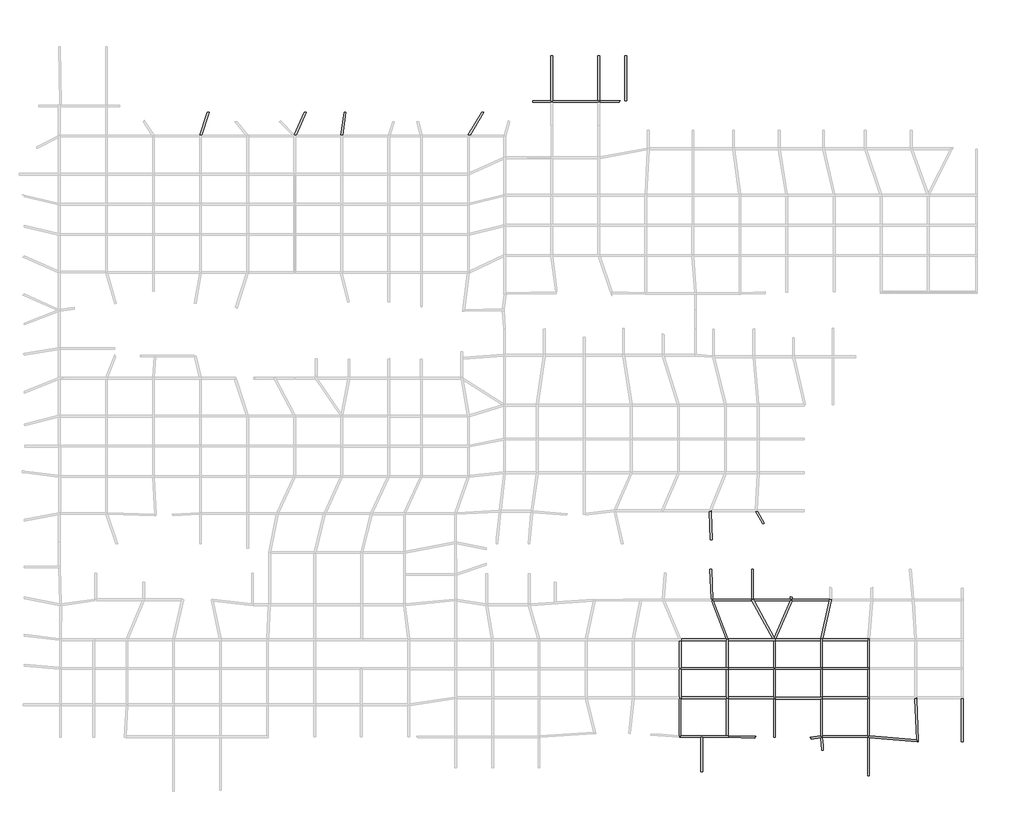
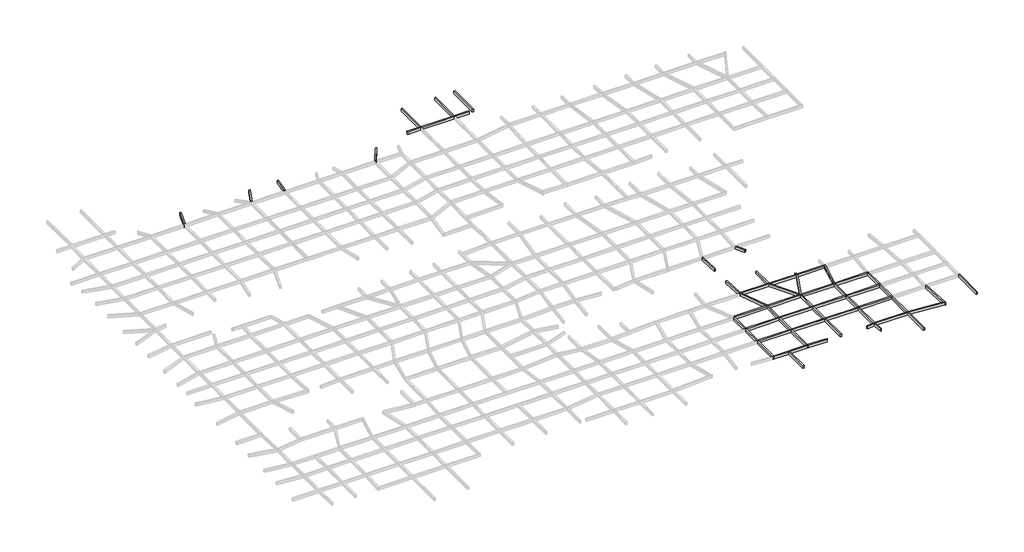
# One storey, part 13 of 15: 59 beams.
"""IFC4 building model written with IfcOpenShell, lengths in millimetres."""

import ifcopenshell
import ifcopenshell.guid

model = None  # the IFC model being written
_history = None  # IfcOwnerHistory: only IFC2X3 demands one
_inside = {}  # id of a spatial element -> (the spatial element, [elements in it])
_under = {}  # id of a project, library or spatial element -> (it, [spatial elements below it])
_declared = {}  # id of a project -> (the project, [libraries it declares])
_typed = {}  # id of a type object -> (the type object, [elements of that type])
_made_of = {}  # id of a material, layer set ... -> (it, [elements and type objects made of it])


def new_model(schema):
    """Start an empty IFC model of exactly this schema.

    Asked for "IFC4X3", IfcOpenShell would pick the latest addendum, in which some entities
    have other attributes; the version numbers below select the first issue.
    IFC2X3 requires an IfcOwnerHistory on every rooted entity: one is made here for all.
    """
    global model, _history
    if schema == "IFC4X3":
        model = ifcopenshell.file(schema_version=(4, 3, 0, 0))
    else:
        model = ifcopenshell.file(schema=schema)
    _inside.clear()
    _under.clear()
    _declared.clear()
    _typed.clear()
    _made_of.clear()
    _history = None
    if model.schema == "IFC2X3":
        org = make("IfcOrganization", Name="unknown")
        user = make(
            "IfcPersonAndOrganization",
            ThePerson=make("IfcPerson", FamilyName="unknown"),
            TheOrganization=org,
        )
        app = make(
            "IfcApplication",
            ApplicationDeveloper=org,
            Version="unknown",
            ApplicationFullName="unknown",
            ApplicationIdentifier="unknown",
        )
        _history = make(
            "IfcOwnerHistory",
            OwningUser=user,
            OwningApplication=app,
            ChangeAction="ADDED",
            CreationDate=0,
        )
    return model


def make(cls, **values):
    """One entity of the class cls with the attributes given. An attribute that is None is left unset."""
    return model.create_entity(
        cls, **{name: value for name, value in values.items() if value is not None}
    )


def rooted(cls, **values):
    """An entity with a GlobalId (a new one), such as an element, a storey or a relation."""
    return make(cls, GlobalId=ifcopenshell.guid.new(), OwnerHistory=_history, **values)


def si_unit(unit_type, name, prefix=None):
    """IfcSIUnit, for example si_unit("LENGTHUNIT", "METRE", prefix="MILLI")."""
    return make("IfcSIUnit", UnitType=unit_type, Prefix=prefix, Name=name)


def assignment(units):
    """IfcUnitAssignment: the units of a project."""
    return None if units is None else make("IfcUnitAssignment", Units=units)


def point(xyz):
    """IfcCartesianPoint."""
    return None if xyz is None else make("IfcCartesianPoint", Coordinates=xyz)


def direction(xyz):
    """IfcDirection."""
    return None if xyz is None else make("IfcDirection", DirectionRatios=xyz)


def frame(location, z_axis=None, x_axis=None):
    """IfcAxis2Placement3D, a coordinate frame: its origin and axes. An axis left out is left unset."""
    return make(
        "IfcAxis2Placement3D",
        Location=point(location),
        Axis=direction(z_axis),
        RefDirection=direction(x_axis),
    )


def origin():
    """The frame at (0, 0, 0) with its axes left unset."""
    return frame((0.0, 0.0, 0.0))


def place(relative_to, where):
    """IfcLocalPlacement: puts the frame where relative to a parent placement (None: the world)."""
    return make(
        "IfcLocalPlacement", PlacementRelTo=relative_to, RelativePlacement=where
    )


def context(
    kind, dimensions, precision=None, world=None, true_north=None, identifier=None
):
    """IfcGeometricRepresentationContext, for example the 3D "Model" context."""
    return make(
        "IfcGeometricRepresentationContext",
        ContextIdentifier=identifier,
        ContextType=kind,
        CoordinateSpaceDimension=dimensions,
        Precision=precision,
        WorldCoordinateSystem=world,
        TrueNorth=true_north,
    )


def project(units=None, contexts=None):
    """IfcProject with its units and contexts."""
    return rooted(
        "IfcProject",
        Name="project",
        RepresentationContexts=contexts,
        UnitsInContext=assignment(units),
    )


def spatial(cls, under=None, at=None, **own):
    """A site, building, storey or space (cls), placed at a placement, below another one or the project."""
    s = rooted(cls, ObjectPlacement=at, **own)
    if under is not None:
        _under.setdefault(under.id(), (under, []))[1].append(s)
    return s


def polyline(points):
    """IfcPolyline through the points."""
    return make("IfcPolyline", Points=[point(p) for p in points])


def outline(outer, holes=None, kind="AREA"):
    """IfcArbitraryClosedProfileDef: a profile drawn as a closed curve; with holes, ...WithVoids."""
    if holes is None:
        return make("IfcArbitraryClosedProfileDef", ProfileType=kind, OuterCurve=outer)
    return make(
        "IfcArbitraryProfileDefWithVoids",
        ProfileType=kind,
        OuterCurve=outer,
        InnerCurves=holes,
    )


def extrude(swept, where, along, depth):
    """IfcExtrudedAreaSolid: the profile swept, set in the frame where, extruded along a direction by depth."""
    return make(
        "IfcExtrudedAreaSolid",
        SweptArea=swept,
        Position=where,
        ExtrudedDirection=direction(along),
        Depth=depth,
    )


def faces_of(points, faces, orient=None, outer=None):
    """IfcFace entities. A face is a list of loops; a loop is a list of indices into points, from 0.

    orient and outer hold one flag for each loop. By default every Orientation is true, the
    first loop of a face is its IfcFaceOuterBound and the others are IfcFaceBound.
    """
    made = []
    for i, loops in enumerate(faces):
        bounds = []
        for j, loop in enumerate(loops):
            is_outer = j == 0 if outer is None else outer[i][j]
            bounds.append(
                make(
                    "IfcFaceOuterBound" if is_outer else "IfcFaceBound",
                    Bound=make("IfcPolyLoop", Polygon=[points[k] for k in loop]),
                    Orientation=True if orient is None else orient[i][j],
                )
            )
        made.append(make("IfcFace", Bounds=bounds))
    return made


def faceted_brep(points, faces, orient=None, outer=None, voids=None):
    """IfcFacetedBrep: a solid bounded by flat faces; with voids (closed shells), ...WithVoids."""
    shared = [point(p) for p in points]
    hull = make("IfcClosedShell", CfsFaces=faces_of(shared, faces, orient, outer))
    if voids is None:
        return make("IfcFacetedBrep", Outer=hull)
    return make(
        "IfcFacetedBrepWithVoids",
        Outer=hull,
        Voids=[
            make(cls, CfsFaces=faces_of(shared, fs, o, b)) for cls, fs, o, b in voids
        ],
    )


def shape(context_of_items, identifier, shape_type, items):
    """IfcShapeRepresentation: the items that make up one representation, for example the "Body"."""
    return make(
        "IfcShapeRepresentation",
        ContextOfItems=context_of_items,
        RepresentationIdentifier=identifier,
        RepresentationType=shape_type,
        Items=items,
    )


def made_of(thing, what):
    """Note that an element or type object is made of a material, layer set ...; save() writes the relation."""
    if what is not None:
        _made_of.setdefault(what.id(), (what, []))[1].append(thing)
    return thing


def element(
    cls,
    number,
    at=None,
    inside=None,
    cuts=None,
    type_object=None,
    material=None,
    context=None,
    identifier="Body",
    shape_type=None,
    held_by="IfcProductDefinitionShape",
    body=None,
    shapes=None,
    **own,
):
    """One element of the class cls, such as IfcWall. Its Tag is "e" and its number.

    at: its placement. inside: the storey or other place that contains it. cuts: it is an
    opening in that element (IfcRelVoidsElement). A single representation is given by context,
    identifier, shape_type and body (its items); several are given by shapes. held_by: the class
    of the entity that holds the representations. save() writes the other relations.
    """
    e = rooted(cls, Tag="e%d" % number, ObjectPlacement=at, **own)
    if body is not None:
        shapes = [shape(context, identifier, shape_type, body)]
    if shapes is not None:
        e.Representation = make(held_by, Representations=shapes)
    if inside is not None:
        _inside.setdefault(inside.id(), (inside, []))[1].append(e)
    if cuts is not None:
        rooted(
            "IfcRelVoidsElement", RelatingBuildingElement=cuts, RelatedOpeningElement=e
        )
    if type_object is not None:
        _typed.setdefault(type_object.id(), (type_object, []))[1].append(e)
    return made_of(e, material)


def aggregate(whole, parts):
    """IfcRelAggregates: a whole, such as a stair, and the parts it consists of."""
    return rooted("IfcRelAggregates", RelatingObject=whole, RelatedObjects=parts)


def save(model, path):
    """Write the relations noted so far, then the file.

    IfcRelAggregates (storeys below a building ...), IfcRelContainedInSpatialStructure (elements
    in a storey), IfcRelDefinesByType, IfcRelAssociatesMaterial and IfcRelDeclares: one each for
    every whole, place, type object, material and project.
    """
    for whole, parts in _under.values():
        aggregate(whole, parts)
    for where, things in _inside.values():
        rooted(
            "IfcRelContainedInSpatialStructure",
            RelatedElements=things,
            RelatingStructure=where,
        )
    for kind, things in _typed.values():
        rooted("IfcRelDefinesByType", RelatedObjects=things, RelatingType=kind)
    for what, things in _made_of.values():
        rooted("IfcRelAssociatesMaterial", RelatedObjects=things, RelatingMaterial=what)
    for by, libraries in _declared.values():
        rooted("IfcRelDeclares", RelatingContext=by, RelatedDefinitions=libraries)
    model.write(path)


model = new_model("IFC4")

# Units and contexts
model_context = context("Model", 3, world=origin())
ifc_project = project(units=[si_unit("LENGTHUNIT", "METRE", prefix="MILLI")], contexts=[model_context])

# Site, building, storey
site = spatial("IfcSite", under=ifc_project)
building = spatial("IfcBuilding", under=site)
storey = spatial("IfcBuildingStorey", under=building, Name="层高", Elevation=3300.0)

# Beams
placement = place(None, origin())
element("IfcBeam", 1, ObjectType="混凝土 - 矩形梁 : KL_beam", at=placement, inside=storey, context=model_context, shape_type="Brep", body=[
    faceted_brep([(256449.8189959, 38242.26105, 3300.0), (256749.8189959, 38242.26105, 3300.0), (256749.8189959, 38542.26105, 3300.0), (256749.8189959, 43042.26105, 3300.0), (256449.8189959, 43042.26105, 3300.0), (256449.8189959, 38542.26105, 3300.0), (256449.8189959, 38242.26105, 2700.0), (256449.8189959, 43042.26105, 2700.0), (256449.8189959, 38542.26105, 2700.0), (256749.8189959, 38242.26105, 2700.0), (256749.8189959, 43042.26105, 2700.0), (256749.8189959, 38542.26105, 2700.0)], [[[0, 1, 2, 3, 4, 5]], [[6, 0, 5, 4, 7, 8]], [[9, 6, 8, 7, 10, 11]], [[1, 9, 11, 10, 3, 2]], [[4, 3, 10, 7]], [[1, 0, 6, 9]]]),
])
element("IfcBeam", 2, ObjectType="混凝土 - 矩形梁 : KL_beam", at=placement, inside=storey, context=model_context, shape_type="Brep", body=[
    faceted_brep([(256449.8189959, 33392.26105, 3300.0), (256705.4878315, 33392.26105, 3300.0), (256749.8189959, 33392.26105, 3300.0), (256749.8189959, 33692.26105, 3300.0), (256749.8189959, 38242.26105, 3300.0), (256449.8189959, 38242.26105, 3300.0), (256449.8189959, 33692.26105, 3300.0), (256749.8189959, 33392.26105, 2700.0), (256749.8189959, 33692.26105, 2700.0), (256749.8189959, 38242.26105, 2700.0), (256705.4878315, 33392.26105, 2700.0), (256449.8189959, 33392.26105, 2700.0), (256449.8189959, 33692.26105, 2700.0), (256449.8189959, 38242.26105, 2700.0)], [[[0, 1, 2, 3, 4, 5, 6]], [[2, 7, 8, 9, 4, 3]], [[7, 10, 11, 12, 13, 9, 8]], [[11, 0, 6, 5, 13, 12]], [[5, 4, 9, 13]], [[2, 1, 0, 11, 10, 7]]]),
])
element("IfcBeam", 3, ObjectType="混凝土 - 矩形梁 : KL_beam", at=placement, inside=storey, context=model_context, shape_type="Brep", body=[
    faceted_brep([(264549.8189959, 38242.26105, 3300.0), (264549.8189959, 38542.26105, 3300.0), (264249.8189959, 38542.26105, 3300.0), (256749.8189959, 38542.26105, 3300.0), (256749.8189959, 38242.26105, 3300.0), (264249.8189959, 38242.26105, 3300.0), (264549.8189959, 38242.26105, 2700.0), (256749.8189959, 38242.26105, 2700.0), (264249.8189959, 38242.26105, 2700.0), (264549.8189959, 38542.26105, 2700.0), (256749.8189959, 38542.26105, 2700.0), (264249.8189959, 38542.26105, 2700.0)], [[[0, 1, 2, 3, 4, 5]], [[6, 0, 5, 4, 7, 8]], [[9, 6, 8, 7, 10, 11]], [[1, 9, 11, 10, 3, 2]], [[4, 3, 10, 7]], [[1, 0, 6, 9]]]),
])
element("IfcBeam", 4, ObjectType="混凝土 - 矩形梁 : KL_beam", at=placement, inside=storey, context=model_context, shape_type="Brep", body=[
    faceted_brep([(264549.8189959, 43342.26105, 3300.0), (264502.8450069, 43342.26105, 3300.0), (264249.8189959, 43342.26105, 3300.0), (264249.8189959, 43042.26105, 3300.0), (264249.8189959, 38542.26105, 3300.0), (264549.8189959, 38542.26105, 3300.0), (264549.8189959, 43042.26105, 3300.0), (264549.8189959, 43342.26105, 2700.0), (264549.8189959, 38542.26105, 2700.0), (264549.8189959, 43042.26105, 2700.0), (264249.8189959, 43342.26105, 2700.0), (264502.8450069, 43342.26105, 2700.0), (264249.8189959, 38542.26105, 2700.0), (264249.8189959, 43042.26105, 2700.0)], [[[0, 1, 2, 3, 4, 5, 6]], [[7, 0, 6, 5, 8, 9]], [[10, 11, 7, 9, 8, 12, 13]], [[2, 10, 13, 12, 4, 3]], [[5, 4, 12, 8]], [[2, 1, 0, 7, 11, 10]]]),
])
element("IfcBeam", 5, ObjectType="混凝土 - 矩形梁 : KL_beam", at=placement, inside=storey, context=model_context, shape_type="Brep", body=[
    faceted_brep([(256749.8189959, 43342.26105, 3300.0), (256749.8189959, 43042.26105, 3300.0), (264249.8189959, 43042.26105, 3300.0), (264249.8189959, 43342.26105, 3300.0), (264181.4275453, 43342.26105, 3300.0), (256749.8189959, 43342.26105, 2700.0), (264249.8189959, 43342.26105, 2700.0), (264181.4275453, 43342.26105, 2700.0), (256749.8189959, 43042.26105, 2700.0), (264249.8189959, 43042.26105, 2700.0)], [[[0, 1, 2, 3, 4]], [[5, 0, 4, 3, 6, 7]], [[8, 5, 7, 6, 9]], [[1, 8, 9, 2]], [[1, 0, 5, 8]], [[3, 2, 9, 6]]]),
])
element("IfcBeam", 6, ObjectType="混凝土 - 矩形梁 : KL_beam", at=placement, inside=storey, context=model_context, shape_type="Brep", body=[
    faceted_brep([(264249.8189959, 33392.26105, 3300.0), (264549.8189959, 33392.26105, 3300.0), (264549.8189959, 33692.2610501, 3300.0), (264549.8189959, 38242.26105, 3300.0), (264249.8189959, 38242.26105, 3300.0), (264249.8189959, 33692.26105, 3300.0), (264249.8189959, 33392.26105, 2700.0), (264249.8189959, 38242.26105, 2700.0), (264249.8189959, 33692.26105, 2700.0), (264549.8189959, 33392.26105, 2700.0), (264549.8189959, 38242.26105, 2700.0), (264549.8189959, 33692.2610501, 2700.0)], [[[0, 1, 2, 3, 4, 5]], [[6, 0, 5, 4, 7, 8]], [[9, 6, 8, 7, 10, 11]], [[1, 9, 11, 10, 3, 2]], [[4, 3, 10, 7]], [[1, 0, 6, 9]]]),
])
element("IfcBeam", 7, ObjectType="混凝土 - 矩形梁 : KL_beam", at=placement, inside=storey, context=model_context, shape_type="SweptSolid", body=[
    extrude(outline(polyline([(256749.8189959, 33392.26105), (256749.8189959, 33692.26105), (264249.8189959, 33692.26105), (264249.8189959, 33392.26105), (256749.8189959, 33392.26105)])), frame((0.0, 0.0, 2700.0), z_axis=(0.0, 0.0, 1.0), x_axis=(1.0, 0.0, 0.0)), (0.0, 0.0, 1.0), 600.0),
])
element("IfcBeam", 8, ObjectType="混凝土 - 矩形梁 : KL_beam", at=placement, inside=storey, context=model_context, shape_type="Brep", body=[
    faceted_brep([(264549.8189959, 43342.26105, 3300.0), (264549.8189959, 43042.26105, 3300.0), (272049.8189959, 43042.26105, 3300.0), (272349.8189959, 43042.26105, 3300.0), (272349.8189959, 43342.26105, 3300.0), (272101.8087649, 43342.26105, 3300.0), (271945.2868475, 43342.26105, 3300.0), (264549.8189959, 43042.26105, 2700.0), (272049.8189959, 43042.26105, 2700.0), (272349.8189959, 43042.26105, 2700.0), (264549.8189959, 43342.26105, 2700.0), (271945.2868475, 43342.26105, 2700.0), (272101.8087649, 43342.26105, 2700.0), (272349.8189959, 43342.26105, 2700.0)], [[[0, 1, 2, 3, 4, 5, 6]], [[1, 7, 8, 9, 3, 2]], [[7, 10, 11, 12, 13, 9, 8]], [[10, 0, 6, 5, 4, 13, 12, 11]], [[1, 0, 10, 7]], [[4, 3, 9, 13]]]),
])
element("IfcBeam", 9, ObjectType="混凝土 - 矩形梁 : KL_beam", at=placement, inside=storey, context=model_context, shape_type="Brep", body=[
    faceted_brep([(272049.8189959, 38242.26105, 3300.0), (272349.8189959, 38242.26105, 3300.0), (272349.8189959, 38542.26105, 3300.0), (272349.8189959, 43042.26105, 3300.0), (272049.8189959, 43042.26105, 3300.0), (272049.8189959, 38542.26105, 3300.0), (272049.8189959, 38242.26105, 2700.0), (272049.8189959, 43042.26105, 2700.0), (272049.8189959, 38542.26105, 2700.0), (272349.8189959, 38242.26105, 2700.0), (272349.8189959, 43042.26105, 2700.0), (272349.8189959, 38542.26105, 2700.0)], [[[0, 1, 2, 3, 4, 5]], [[6, 0, 5, 4, 7, 8]], [[9, 6, 8, 7, 10, 11]], [[1, 9, 11, 10, 3, 2]], [[4, 3, 10, 7]], [[1, 0, 6, 9]]]),
])
element("IfcBeam", 10, ObjectType="混凝土 - 矩形梁 : KL_beam", at=placement, inside=storey, context=model_context, shape_type="Brep", body=[
    faceted_brep([(272049.8189959, 33392.2610501, 3300.0), (272349.8189959, 33392.2610501, 3300.0), (272349.8189959, 33642.26105, 3300.0), (272349.8189959, 38242.26105, 3300.0), (272049.8189959, 38242.26105, 3300.0), (272049.8189959, 33692.2610501, 3300.0), (272049.8189959, 33392.2610501, 2700.0), (272049.8189959, 38242.26105, 2700.0), (272049.8189959, 33692.2610501, 2700.0), (272349.8189959, 33392.2610501, 2700.0), (272349.8189959, 38242.26105, 2700.0), (272349.8189959, 33642.26105, 2700.0)], [[[0, 1, 2, 3, 4, 5]], [[6, 0, 5, 4, 7, 8]], [[9, 6, 8, 7, 10, 11]], [[1, 9, 11, 10, 3, 2]], [[4, 3, 10, 7]], [[1, 0, 6, 9]]]),
])
element("IfcBeam", 11, ObjectType="混凝土 - 矩形梁 : KL_beam", at=placement, inside=storey, context=model_context, shape_type="SweptSolid", body=[
    extrude(outline(polyline([(264549.8189959, 38242.26105), (264549.8189959, 38542.26105), (272049.8189959, 38542.26105), (272049.8189959, 38242.26105), (264549.8189959, 38242.26105)])), frame((0.0, 0.0, 2700.0), z_axis=(0.0, 0.0, 1.0), x_axis=(1.0, 0.0, 0.0)), (0.0, 0.0, 1.0), 600.0),
])
element("IfcBeam", 12, ObjectType="混凝土 - 矩形梁 : KL_beam", at=placement, inside=storey, context=model_context, shape_type="SweptSolid", body=[
    extrude(outline(polyline([(264549.8189959, 33392.2610501), (264549.8189959, 33692.2610501), (272049.8189959, 33692.2610501), (272049.8189959, 33392.2610501), (264549.8189959, 33392.2610501)])), frame((0.0, 0.0, 2700.0), z_axis=(0.0, 0.0, 1.0), x_axis=(1.0, 0.0, 0.0)), (0.0, 0.0, 1.0), 600.0),
])
element("IfcBeam", 13, ObjectType="混凝土 - 矩形梁 : KL_beam", at=placement, inside=storey, context=model_context, shape_type="Brep", body=[
    faceted_brep([(280149.8189959, 38242.26105, 3300.0), (280149.8189959, 38542.26105, 3300.0), (279849.8189959, 38542.26105, 3300.0), (272349.8189959, 38542.26105, 3300.0), (272349.8189959, 38242.26105, 3300.0), (279849.8189959, 38242.26105, 3300.0), (280149.8189959, 38242.26105, 2700.0), (272349.8189959, 38242.26105, 2700.0), (279849.8189959, 38242.26105, 2700.0), (280149.8189959, 38542.26105, 2700.0), (272349.8189959, 38542.26105, 2700.0), (279849.8189959, 38542.26105, 2700.0)], [[[0, 1, 2, 3, 4, 5]], [[6, 0, 5, 4, 7, 8]], [[9, 6, 8, 7, 10, 11]], [[1, 9, 11, 10, 3, 2]], [[4, 3, 10, 7]], [[1, 0, 6, 9]]]),
])
element("IfcBeam", 14, ObjectType="混凝土 - 矩形梁 : KL_beam", at=placement, inside=storey, context=model_context, shape_type="Brep", body=[
    faceted_brep([(272049.8189959, 33392.2610501, 3300.0), (272049.8189959, 33342.26105, 3300.0), (272349.8189959, 33342.26105, 3300.0), (279849.8189959, 33342.26105, 3300.0), (280149.8189959, 33342.26105, 3300.0), (280149.8189959, 33392.26105, 3300.0), (280149.8189959, 33642.26105, 3300.0), (279849.8189959, 33642.26105, 3300.0), (272349.8189959, 33642.26105, 3300.0), (272349.8189959, 33392.2610501, 3300.0), (272349.8189959, 33642.26105, 2700.0), (280149.8189959, 33642.26105, 2700.0), (279849.8189959, 33642.26105, 2700.0), (272049.8189959, 33342.26105, 2700.0), (272049.8189959, 33392.2610501, 2700.0), (272349.8189959, 33392.2610501, 2700.0), (280149.8189959, 33392.26105, 2700.0), (280149.8189959, 33342.26105, 2700.0), (279849.8189959, 33342.26105, 2700.0), (272349.8189959, 33342.26105, 2700.0)], [[[0, 1, 2, 3, 4, 5, 6, 7, 8, 9]], [[10, 8, 7, 6, 11, 12]], [[13, 14, 15, 10, 12, 11, 16, 17, 18, 19]], [[1, 13, 19, 18, 17, 4, 3, 2]], [[13, 1, 0, 14]], [[15, 9, 8, 10]], [[9, 15, 14, 0]], [[6, 5, 4, 17, 16, 11]]]),
])
element("IfcBeam", 15, ObjectType="混凝土 - 矩形梁 : KL_beam", at=placement, inside=storey, context=model_context, shape_type="Brep", body=[
    faceted_brep([(287949.8189959, 38242.26105, 3300.0), (287949.8189959, 38542.26105, 3300.0), (287649.8189959, 38542.26105, 3300.0), (280149.8189959, 38542.26105, 3300.0), (280149.8189959, 38242.26105, 3300.0), (287649.8189959, 38242.26105, 3300.0), (287949.8189959, 38242.26105, 2700.0), (280149.8189959, 38242.26105, 2700.0), (287649.8189959, 38242.26105, 2700.0), (287949.8189959, 38542.26105, 2700.0), (280149.8189959, 38542.26105, 2700.0), (287649.8189959, 38542.26105, 2700.0)], [[[0, 1, 2, 3, 4, 5]], [[6, 0, 5, 4, 7, 8]], [[9, 6, 8, 7, 10, 11]], [[1, 9, 11, 10, 3, 2]], [[1, 0, 6, 9]], [[4, 3, 10, 7]]]),
])
element("IfcBeam", 16, ObjectType="混凝土 - 矩形梁 : KL_beam", at=placement, inside=storey, context=model_context, shape_type="Brep", body=[
    faceted_brep([(287649.8189959, 33392.26105, 3300.0), (287949.8189959, 33392.26105, 3300.0), (287949.8189959, 33692.26105, 3300.0), (287949.8189959, 38242.26105, 3300.0), (287649.8189959, 38242.26105, 3300.0), (287649.8189959, 33692.26105, 3300.0), (287649.8189959, 33392.26105, 2700.0), (287649.8189959, 38242.26105, 2700.0), (287649.8189959, 33692.26105, 2700.0), (287949.8189959, 33392.26105, 2700.0), (287949.8189959, 38242.26105, 2700.0), (287949.8189959, 33692.26105, 2700.0)], [[[0, 1, 2, 3, 4, 5]], [[6, 0, 5, 4, 7, 8]], [[9, 6, 8, 7, 10, 11]], [[1, 9, 11, 10, 3, 2]], [[4, 3, 10, 7]], [[1, 0, 6, 9]]]),
])
element("IfcBeam", 17, ObjectType="混凝土 - 矩形梁 : KL_beam", at=placement, inside=storey, context=model_context, shape_type="Brep", body=[
    faceted_brep([(287649.8189959, 33392.26105, 3300.0), (287649.8189959, 33692.26105, 3300.0), (280149.8189959, 33692.26105, 3300.0), (279849.8189959, 33692.26105, 3300.0), (279849.8189959, 33642.26105, 3300.0), (280149.8189959, 33642.26105, 3300.0), (280149.8189959, 33392.26105, 3300.0), (287649.8189959, 33692.26105, 2700.0), (280149.8189959, 33692.26105, 2700.0), (279849.8189959, 33692.26105, 2700.0), (287649.8189959, 33392.26105, 2700.0), (280149.8189959, 33392.26105, 2700.0), (280149.8189959, 33642.26105, 2700.0), (279849.8189959, 33642.26105, 2700.0)], [[[0, 1, 2, 3, 4, 5, 6]], [[1, 7, 8, 9, 3, 2]], [[7, 10, 11, 12, 13, 9, 8]], [[10, 0, 6, 11]], [[12, 5, 4, 13]], [[7, 1, 0, 10]], [[3, 9, 13, 4]], [[5, 12, 11, 6]]]),
])
element("IfcBeam", 18, ObjectType="混凝土 - 矩形梁 : KL_beam", at=placement, inside=storey, context=model_context, shape_type="Brep", body=[
    faceted_brep([(295769.3386413, 26348.7115862, 3300.0), (295855.5253292, 26346.5943052, 3300.0), (295858.4723864, 26466.5581116, 3300.0), (296064.6228807, 26461.4937733, 3300.0), (295756.6327439, 33392.26105, 3300.0), (295749.8189959, 33545.5922638, 3300.0), (295749.8189959, 33392.26105, 3300.0), (295456.3366783, 33392.26105, 3300.0), (295759.529407, 26569.4508639, 3300.0), (295769.3386413, 26348.7115862, 2700.0), (295456.3366783, 33392.26105, 2700.0), (295759.529407, 26569.4508639, 2700.0), (295855.5253292, 26346.5943052, 2700.0), (295749.8189959, 33392.26105, 2700.0), (295749.8189959, 33545.5922638, 2700.0), (295756.6327439, 33392.26105, 2700.0), (296064.6228807, 26461.4937733, 2700.0), (295858.4723864, 26466.5581116, 2700.0)], [[[0, 1, 2, 3, 4, 5, 6, 7, 8]], [[9, 0, 8, 7, 10, 11]], [[12, 9, 11, 10, 13, 14, 15, 16, 17]], [[14, 5, 4, 3, 16, 15]], [[0, 9, 12, 1]], [[17, 2, 1, 12]], [[2, 17, 16, 3]], [[13, 6, 5, 14]], [[6, 13, 10, 7]]]),
])
element("IfcBeam", 19, ObjectType="混凝土 - 矩形梁 : KL_beam", at=placement, inside=storey, context=model_context, shape_type="Brep", body=[
    faceted_brep([(295853.4003013, 26260.0922736, 3300.0), (295855.5253292, 26346.5943052, 3300.0), (295769.3386413, 26348.7115862, 3300.0), (295759.529407, 26569.4508639, 3300.0), (287949.8189959, 27252.7119903, 3300.0), (287649.8189959, 27278.9585894, 3300.0), (287649.8189959, 26992.26105, 3300.0), (287649.8189959, 26977.8126381, 3300.0), (287949.8189959, 26951.5660391, 3300.0), (295759.529407, 26569.4508639, 2700.0), (287949.8189959, 27252.7119903, 2700.0), (287649.8189959, 27278.9585894, 2700.0), (295855.5253292, 26346.5943052, 2700.0), (295853.4003013, 26260.0922736, 2700.0), (287949.8189959, 26951.5660391, 2700.0), (287649.8189959, 26977.8126381, 2700.0), (287649.8189959, 26992.26105, 2700.0), (295769.3386413, 26348.7115862, 2700.0)], [[[0, 1, 2, 3, 4, 5, 6, 7, 8]], [[3, 9, 10, 11, 5, 4]], [[12, 13, 14, 15, 16, 11, 10, 9, 17]], [[13, 0, 8, 7, 15, 14]], [[0, 13, 12, 1]], [[2, 17, 9, 3]], [[17, 2, 1, 12]], [[7, 6, 5, 11, 16, 15]]]),
    faceted_brep([(296074.4321151, 26240.7544956, 3300.0), (296074.4321151, 26240.7544956, 2700.0), (296069.9628913, 26341.326385, 2700.0), (296069.9628913, 26341.326385, 3300.0), (295973.1790694, 26249.6129893, 2700.0), (295973.1790694, 26249.6129893, 3300.0), (295975.4891356, 26343.647248, 3300.0), (295975.4891356, 26343.647248, 2700.0)], [[[0, 1, 2, 3]], [[4, 5, 6, 7]], [[1, 0, 5, 4]], [[6, 5, 0, 3]], [[2, 1, 4, 7]], [[6, 3, 2, 7]]]),
])
element("IfcBeam", 20, ObjectType="混凝土 - 矩形梁 : KL_beam", at=placement, inside=storey, context=model_context, shape_type="Brep", body=[
    faceted_brep([(287949.8189959, 33392.26105, 3300.0), (287649.8189959, 33392.26105, 3300.0), (287649.8189959, 27292.26105, 3300.0), (287649.8189959, 27278.9585894, 3300.0), (287949.8189959, 27252.7119903, 3300.0), (287949.8189959, 33392.26105, 2700.0), (287949.8189959, 27252.7119903, 2700.0), (287649.8189959, 33392.26105, 2700.0), (287649.8189959, 27278.9585894, 2700.0), (287649.8189959, 27292.26105, 2700.0)], [[[0, 1, 2, 3, 4]], [[5, 0, 4, 6]], [[7, 5, 6, 8, 9]], [[1, 7, 9, 8, 3, 2]], [[1, 0, 5, 7]], [[4, 3, 8, 6]]]),
])
element("IfcBeam", 21, ObjectType="混凝土 - 矩形梁 : KL_beam", at=placement, inside=storey, context=model_context, shape_type="Brep", body=[
    faceted_brep([(279849.8189959, 26992.26105, 3300.0), (280012.5168324, 26992.26105, 3300.0), (280149.8189959, 26992.26105, 3300.0), (280149.8189959, 27292.26105, 3300.0), (280149.8189959, 33342.26105, 3300.0), (279849.8189959, 33342.26105, 3300.0), (279849.8189959, 27268.8473955, 3300.0), (280149.8189959, 26992.26105, 2700.0), (280149.8189959, 27292.26105, 2700.0), (280149.8189959, 33342.26105, 2700.0), (280012.5168324, 26992.26105, 2700.0), (279849.8189959, 26992.26105, 2700.0), (279849.8189959, 27268.8473955, 2700.0), (279849.8189959, 33342.26105, 2700.0)], [[[0, 1, 2, 3, 4, 5, 6]], [[2, 7, 8, 9, 4, 3]], [[7, 10, 11, 12, 13, 9, 8]], [[11, 0, 6, 5, 13, 12]], [[5, 4, 9, 13]], [[2, 1, 0, 11, 10, 7]]]),
])
element("IfcBeam", 22, ObjectType="混凝土 - 矩形梁 : KL_beam", at=placement, inside=storey, context=model_context, shape_type="Brep", body=[
    faceted_brep([(280149.8189959, 27292.26105, 3300.0), (280149.8189959, 26992.26105, 3300.0), (280164.0010329, 26992.26105, 3300.0), (287649.8189959, 26992.26105, 3300.0), (287649.8189959, 27278.9585894, 3300.0), (287649.8189959, 27292.26105, 3300.0), (280149.8189959, 26992.26105, 2700.0), (280164.0010329, 26992.26105, 2700.0), (287649.8189959, 26992.26105, 2700.0), (280149.8189959, 27292.26105, 2700.0), (287649.8189959, 27292.26105, 2700.0), (287649.8189959, 27278.9585894, 2700.0)], [[[0, 1, 2, 3, 4, 5]], [[1, 6, 7, 8, 3, 2]], [[6, 9, 10, 11, 8, 7]], [[9, 0, 5, 10]], [[1, 0, 9, 6]], [[5, 4, 3, 8, 11, 10]]]),
])
element("IfcBeam", 23, ObjectType="混凝土 - 矩形梁 : KL_beam", at=placement, inside=storey, context=model_context, shape_type="SweptSolid", body=[
    extrude(outline(polyline([(279849.8189959, 38242.26105), (280149.8189959, 38242.26105), (280149.8189959, 33692.26105), (279849.8189959, 33692.26105), (279849.8189959, 38242.26105)])), frame((0.0, 0.0, 2700.0), z_axis=(0.0, 0.0, 1.0), x_axis=(1.0, 0.0, 0.0)), (0.0, 0.0, 1.0), 600.0),
])
element("IfcBeam", 24, ObjectType="混凝土 - 矩形梁 : KL_beam", at=placement, inside=storey, context=model_context, shape_type="Brep", body=[
    faceted_brep([(280149.8189959, 43342.26105, 3300.0), (279880.4995347, 43342.26105, 3300.0), (279849.8189959, 43342.26105, 3300.0), (279849.8189959, 43042.26105, 3300.0), (279849.8189959, 38542.26105, 3300.0), (280149.8189959, 38542.26105, 3300.0), (280149.8189959, 43042.26105, 3300.0), (280149.8189959, 43175.1732362, 3300.0), (279849.8189959, 43342.26105, 2700.0), (279849.8189959, 43042.26105, 2700.0), (279849.8189959, 38542.26105, 2700.0), (279880.4995347, 43342.26105, 2700.0), (280149.8189959, 43342.26105, 2700.0), (280149.8189959, 43175.1732362, 2700.0), (280149.8189959, 43042.26105, 2700.0), (280149.8189959, 38542.26105, 2700.0)], [[[0, 1, 2, 3, 4, 5, 6, 7]], [[2, 8, 9, 10, 4, 3]], [[8, 11, 12, 13, 14, 15, 10, 9]], [[12, 0, 7, 6, 5, 15, 14, 13]], [[5, 4, 10, 15]], [[2, 1, 0, 12, 11, 8]]]),
])
element("IfcBeam", 25, ObjectType="混凝土 - 矩形梁 : KL_beam", at=placement, inside=storey, context=model_context, shape_type="Brep", body=[
    faceted_brep([(272349.8189959, 43342.26105, 3300.0), (272349.8189959, 43042.26105, 3300.0), (279849.8189959, 43042.26105, 3300.0), (279849.8189959, 43342.26105, 3300.0), (272429.3868661, 43342.26105, 3300.0), (272349.8189959, 43042.26105, 2700.0), (279849.8189959, 43042.26105, 2700.0), (272349.8189959, 43342.26105, 2700.0), (272429.3868661, 43342.26105, 2700.0), (279849.8189959, 43342.26105, 2700.0)], [[[0, 1, 2, 3, 4]], [[1, 5, 6, 2]], [[5, 7, 8, 9, 6]], [[7, 0, 4, 3, 9, 8]], [[1, 0, 7, 5]], [[3, 2, 6, 9]]]),
])
element("IfcBeam", 26, ObjectType="混凝土 - 矩形梁 : KL_beam", at=placement, inside=storey, context=model_context, shape_type="Brep", body=[
    faceted_brep([(281686.9520176, 49834.2385082, 3300.0), (281633.2776757, 49601.7141002, 3300.0), (280188.3884025, 43342.26105, 3300.0), (280149.8189959, 43175.1732362, 3300.0), (280149.8189959, 43175.1732362, 2700.0), (280188.3884025, 43342.26105, 2700.0), (281633.2776757, 49601.7141002, 2700.0), (281686.9520176, 49834.2385082, 2700.0), (280149.8189959, 43342.26105, 3300.0), (280149.8189959, 43342.26105, 2700.0), (279880.4995347, 43342.26105, 3300.0), (279880.4995347, 43342.26105, 2700.0), (281394.6387533, 49901.7141002, 3300.0), (281325.3888079, 49601.7141002, 3300.0), (281394.6387533, 49901.7141002, 2700.0), (281325.3888079, 49601.7141002, 2700.0)], [[[0, 1, 2, 3, 4, 5, 6, 7]], [[8, 9, 4, 3]], [[9, 8, 10, 11]], [[3, 2, 1, 0, 12, 13, 10, 8]], [[10, 13, 12, 14, 15, 11]], [[11, 15, 14, 7, 6, 5, 4, 9]], [[0, 7, 14, 12]]]),
])
element("IfcBeam", 27, ObjectType="混凝土 - 矩形梁 : KL_beam", at=placement, inside=storey, context=model_context, shape_type="Brep", body=[
    faceted_brep([(274978.2959558, 49901.7141002, 3300.0), (274846.7383166, 49601.7141002, 3300.0), (275174.3164179, 49601.7141002, 3300.0), (281325.3888079, 49601.7141002, 3300.0), (281394.6387533, 49901.7141002, 3300.0), (281363.9582145, 49901.7141002, 3300.0), (275149.8189959, 49901.7141002, 3300.0), (274846.7383166, 49601.7141002, 2700.0), (275174.3164179, 49601.7141002, 2700.0), (281325.3888079, 49601.7141002, 2700.0), (274978.2959558, 49901.7141002, 2700.0), (275149.8189959, 49901.7141002, 2700.0), (281363.9582145, 49901.7141002, 2700.0), (281394.6387533, 49901.7141002, 2700.0)], [[[0, 1, 2, 3, 4, 5, 6]], [[1, 7, 8, 9, 3, 2]], [[7, 10, 11, 12, 13, 9, 8]], [[10, 0, 6, 5, 4, 13, 12, 11]], [[4, 3, 9, 13]], [[1, 0, 10, 7]]]),
])
element("IfcBeam", 28, ObjectType="混凝土 - 矩形梁 : KL_beam", at=placement, inside=storey, context=model_context, shape_type="Brep", body=[
    faceted_brep([(272101.8087649, 43342.26105, 3300.0), (272349.8189959, 43342.26105, 3300.0), (272429.3868661, 43342.26105, 3300.0), (275174.3164179, 49601.7141002, 3300.0), (274846.7383166, 49601.7141002, 3300.0), (272184.1869699, 43530.113779, 3300.0), (272101.8087649, 43342.26105, 2700.0), (274846.7383166, 49601.7141002, 2700.0), (272184.1869699, 43530.113779, 2700.0), (272429.3868661, 43342.26105, 2700.0), (272349.8189959, 43342.26105, 2700.0), (275174.3164179, 49601.7141002, 2700.0)], [[[0, 1, 2, 3, 4, 5]], [[6, 0, 5, 4, 7, 8]], [[9, 10, 6, 8, 7, 11]], [[2, 9, 11, 3]], [[0, 6, 10, 9, 2, 1]], [[4, 3, 11, 7]]]),
])
element("IfcBeam", 29, ObjectType="混凝土 - 矩形梁 : KL_beam", at=placement, inside=storey, context=model_context, shape_type="Brep", body=[
    faceted_brep([(271945.2868475, 43342.26105, 3300.0), (268478.91295, 49601.7141002, 3300.0), (268393.2633896, 49756.3769894, 3300.0), (268393.2633896, 49756.3769894, 2700.0), (268478.91295, 49601.7141002, 2700.0), (271945.2868475, 43342.26105, 2700.0), (272049.8189959, 43342.26105, 2700.0), (272101.8087649, 43342.26105, 2700.0), (272101.8087649, 43342.26105, 3300.0), (272049.8189959, 43342.26105, 3300.0), (272184.1869699, 43530.113779, 3300.0), (268821.8425764, 49601.7141002, 3300.0), (268655.7079061, 49901.7141002, 3300.0), (268655.7079061, 49901.7141002, 2700.0), (268821.8425764, 49601.7141002, 2700.0), (272184.1869699, 43530.113779, 2700.0)], [[[0, 1, 2, 3, 4, 5]], [[0, 5, 6, 7, 8, 9]], [[2, 1, 0, 9, 8, 10, 11, 12]], [[5, 4, 3, 13, 14, 15, 7, 6]], [[13, 12, 11, 10, 15, 14]], [[8, 7, 15, 10]], [[12, 13, 3, 2]]]),
])
element("IfcBeam", 30, ObjectType="混凝土 - 矩形梁 : KL_beam", at=placement, inside=storey, context=model_context, shape_type="Brep", body=[
    faceted_brep([(274978.2959558, 49901.7141002, 3300.0), (274849.8189959, 49901.7141002, 3300.0), (268717.310428, 49901.7141002, 3300.0), (268655.7079061, 49901.7141002, 3300.0), (268821.8425764, 49601.7141002, 3300.0), (274846.7383166, 49601.7141002, 3300.0), (274846.7383166, 49601.7141002, 2700.0), (268821.8425764, 49601.7141002, 2700.0), (268655.7079061, 49901.7141002, 2700.0), (268717.310428, 49901.7141002, 2700.0), (274849.8189959, 49901.7141002, 2700.0), (274978.2959558, 49901.7141002, 2700.0)], [[[0, 1, 2, 3, 4, 5]], [[6, 5, 4, 7]], [[8, 9, 10, 11, 6, 7]], [[3, 2, 1, 0, 11, 10, 9, 8]], [[0, 5, 6, 11]], [[4, 3, 8, 7]]]),
])
element("IfcBeam", 31, ObjectType="混凝土 - 矩形梁 : KL_beam", at=placement, inside=storey, context=model_context, shape_type="Brep", body=[
    faceted_brep([(268478.91295, 49601.7141002, 3300.0), (262095.7631641, 49601.7141002, 3300.0), (261774.3457024, 49601.7141002, 3300.0), (261774.3457024, 49601.7141002, 2700.0), (262095.7631641, 49601.7141002, 2700.0), (268478.91295, 49601.7141002, 2700.0), (261774.3457024, 49901.7141002, 2700.0), (261774.3457024, 49901.7141002, 3300.0), (262020.8281319, 49901.7141002, 3300.0), (268417.310428, 49901.7141002, 3300.0), (268655.7079061, 49901.7141002, 3300.0), (268655.7079061, 49901.7141002, 2700.0), (268417.310428, 49901.7141002, 2700.0), (262020.8281319, 49901.7141002, 2700.0), (268393.2633896, 49756.3769894, 2700.0), (268393.2633896, 49756.3769894, 3300.0)], [[[0, 1, 2, 3, 4, 5]], [[6, 7, 8, 9, 10, 11, 12, 13]], [[14, 15, 0, 5]], [[15, 14, 11, 10]], [[7, 6, 3, 2]], [[2, 1, 0, 15, 10, 9, 8, 7]], [[5, 4, 3, 6, 13, 12, 11, 14]]]),
])
element("IfcBeam", 32, ObjectType="混凝土 - 矩形梁 : KL_beam", at=placement, inside=storey, context=model_context, shape_type="Brep", body=[
    faceted_brep([(261774.3457024, 49601.7141002, 3300.0), (264181.4275453, 43342.26105, 3300.0), (264249.8189959, 43342.26105, 3300.0), (264502.8450069, 43342.26105, 3300.0), (262095.7631641, 49601.7141002, 3300.0), (264502.8450069, 43342.26105, 2700.0), (262095.7631641, 49601.7141002, 2700.0), (264181.4275453, 43342.26105, 2700.0), (261774.3457024, 49601.7141002, 2700.0), (264249.8189959, 43342.26105, 2700.0)], [[[0, 1, 2, 3, 4]], [[3, 5, 6, 4]], [[7, 8, 6, 5, 9]], [[1, 0, 8, 7]], [[5, 3, 2, 1, 7, 9]], [[0, 4, 6, 8]]]),
])
element("IfcBeam", 33, ObjectType="混凝土 - 矩形梁 : KL_beam", at=placement, inside=storey, context=model_context, shape_type="Brep", body=[
    faceted_brep([(261720.5296547, 49901.7141002, 3300.0), (261774.3457024, 49901.7141002, 3300.0), (262020.8281319, 49901.7141002, 3300.0), (261800.8301993, 54832.3246977, 3300.0), (261500.5317222, 54832.3246977, 3300.0), (261720.5296547, 49901.7141002, 2700.0), (261500.5317222, 54832.3246977, 2700.0), (262020.8281319, 49901.7141002, 2700.0), (261774.3457024, 49901.7141002, 2700.0), (261800.8301993, 54832.3246977, 2700.0)], [[[0, 1, 2, 3, 4]], [[5, 0, 4, 6]], [[7, 8, 5, 6, 9]], [[2, 7, 9, 3]], [[7, 2, 1, 0, 5, 8]], [[4, 3, 9, 6]]]),
])
element("IfcBeam", 34, ObjectType="混凝土 - 矩形梁 : KL_beam", at=placement, inside=storey, context=model_context, shape_type="Brep", body=[
    faceted_brep([(268417.310428, 49901.7141002, 3300.0), (268655.7079061, 49901.7141002, 3300.0), (268717.310428, 49901.7141002, 3300.0), (268717.310428, 54832.3246977, 3300.0), (268417.310428, 54832.3246977, 3300.0), (268717.310428, 49901.7141002, 2700.0), (268717.310428, 54832.3246977, 2700.0), (268655.7079061, 49901.7141002, 2700.0), (268417.310428, 49901.7141002, 2700.0), (268417.310428, 54832.3246977, 2700.0)], [[[0, 1, 2, 3, 4]], [[2, 5, 6, 3]], [[5, 7, 8, 9, 6]], [[8, 0, 4, 9]], [[5, 2, 1, 0, 8, 7]], [[4, 3, 6, 9]]]),
])
element("IfcBeam", 35, ObjectType="混凝土 - 矩形梁 : KL_beam", at=placement, inside=storey, context=model_context, shape_type="Brep", body=[
    faceted_brep([(256705.4878315, 33392.26105, 3300.0), (256449.8189959, 33392.26105, 3300.0), (256405.4878315, 33392.26105, 3300.0), (256405.4878315, 27303.3066396, 3300.0), (256405.4878315, 27002.5490588, 3300.0), (256405.4878315, 26992.26105, 3300.0), (256705.4878315, 26992.26105, 3300.0), (256705.4878315, 27292.26105, 3300.0), (256705.4878315, 33392.26105, 2700.0), (256705.4878315, 26992.26105, 2700.0), (256705.4878315, 27292.26105, 2700.0), (256405.4878315, 33392.26105, 2700.0), (256449.8189959, 33392.26105, 2700.0), (256405.4878315, 26992.26105, 2700.0), (256405.4878315, 27002.5490588, 2700.0), (256405.4878315, 27303.3066396, 2700.0)], [[[0, 1, 2, 3, 4, 5, 6, 7]], [[8, 0, 7, 6, 9, 10]], [[11, 12, 8, 10, 9, 13, 14, 15]], [[13, 5, 4, 3, 2, 11, 15, 14]], [[0, 8, 12, 11, 2, 1]], [[6, 5, 13, 9]]]),
])
element("IfcBeam", 36, ObjectType="混凝土 - 矩形梁 : KL_beam", at=placement, inside=storey, context=model_context, shape_type="Brep", body=[
    faceted_brep([(264549.8189959, 26992.26105, 3300.0), (264549.8189959, 27288.6213727, 3300.0), (264549.8189959, 27292.26105, 3300.0), (264249.8189959, 27292.26105, 3300.0), (256705.4878315, 27292.26105, 3300.0), (256705.4878315, 26992.26105, 3300.0), (260005.4878315, 26992.26105, 3300.0), (260305.4878315, 26992.26105, 3300.0), (264397.9768074, 26992.26105, 3300.0), (264549.8189959, 26992.26105, 2700.0), (256705.4878315, 26992.26105, 2700.0), (260005.4878315, 26992.26105, 2700.0), (260305.4878315, 26992.26105, 2700.0), (264397.9768074, 26992.26105, 2700.0), (264549.8189959, 27292.26105, 2700.0), (264549.8189959, 27288.6213727, 2700.0), (256705.4878315, 27292.26105, 2700.0), (264249.8189959, 27292.26105, 2700.0)], [[[0, 1, 2, 3, 4, 5, 6, 7, 8]], [[9, 0, 8, 7, 6, 5, 10, 11, 12, 13]], [[14, 15, 9, 13, 12, 11, 10, 16, 17]], [[2, 14, 17, 16, 4, 3]], [[5, 4, 16, 10]], [[2, 1, 0, 9, 15, 14]]]),
])
element("IfcBeam", 37, ObjectType="混凝土 - 矩形梁 : KL_beam", at=placement, inside=storey, context=model_context, shape_type="SweptSolid", body=[
    extrude(outline(polyline([(264249.8189959, 33392.26105), (264549.8189959, 33392.26105), (264549.8189959, 27292.26105), (264249.8189959, 27292.26105), (264249.8189959, 33392.26105)])), frame((0.0, 0.0, 2700.0), z_axis=(0.0, 0.0, 1.0), x_axis=(1.0, 0.0, 0.0)), (0.0, 0.0, 1.0), 600.0),
])
element("IfcBeam", 38, ObjectType="混凝土 - 矩形梁 : KL_beam", at=placement, inside=storey, context=model_context, shape_type="SweptSolid", body=[
    extrude(outline(polyline([(272349.8189959, 27043.5970722), (272049.8189959, 27050.966938), (272049.8189959, 33342.26105), (272349.8189959, 33342.26105), (272349.8189959, 27043.5970722)])), frame((0.0, 0.0, 2700.0), z_axis=(0.0, 0.0, 1.0), x_axis=(1.0, 0.0, 0.0)), (0.0, 0.0, 1.0), 600.0),
])
element("IfcBeam", 39, ObjectType="混凝土 - 矩形梁 : KL_beam", at=placement, inside=storey, context=model_context, shape_type="SweptSolid", body=[
    extrude(outline(polyline([(269088.6991539, 27177.1182475), (269087.3879177, 27123.7426694), (268967.4241113, 27126.6897266), (268961.3677045, 26880.1557886), (264397.9768074, 26992.26105), (264549.8189959, 26992.26105), (264549.8189959, 27288.6213727), (269088.6991539, 27177.1182475)])), frame((0.0, 0.0, 2700.0), z_axis=(0.0, 0.0, 1.0), x_axis=(1.0, 0.0, 0.0)), (0.0, 0.0, 1.0), 600.0),
])
element("IfcBeam", 40, ObjectType="混凝土 - 矩形梁 : KL_beam", at=placement, inside=storey, context=model_context, shape_type="Brep", body=[
    faceted_brep([(278166.6409107, 26981.8209623, 3300.0), (278164.6492712, 26900.7486766, 3300.0), (278284.6130776, 26897.8016195, 3300.0), (278279.6743809, 26696.7655273, 3300.0), (279865.0508599, 26967.1141969, 3300.0), (280012.5168324, 26992.26105, 3300.0), (279849.8189959, 26992.26105, 3300.0), (279849.8189959, 27268.8473955, 3300.0), (278166.6409107, 26981.8209623, 2700.0), (279849.8189959, 27268.8473955, 2700.0), (278164.6492712, 26900.7486766, 2700.0), (279849.8189959, 26992.26105, 2700.0), (280012.5168324, 26992.26105, 2700.0), (279865.0508599, 26967.1141969, 2700.0), (278279.6743809, 26696.7655273, 2700.0), (278284.6130776, 26897.8016195, 2700.0)], [[[0, 1, 2, 3, 4, 5, 6, 7]], [[8, 0, 7, 9]], [[10, 8, 9, 11, 12, 13, 14, 15]], [[12, 5, 4, 3, 14, 13]], [[0, 8, 10, 1]], [[15, 2, 1, 10]], [[2, 15, 14, 3]], [[6, 11, 9, 7]], [[11, 6, 5, 12]]]),
])
element("IfcBeam", 41, ObjectType="混凝土 - 矩形梁 : KL_beam", at=placement, inside=storey, context=model_context, shape_type="Brep", body=[
    faceted_brep([(280274.041695, 24848.7995976, 3300.0), (280291.9520929, 25577.8657049, 3300.0), (280164.0010329, 26992.26105, 3300.0), (280149.8189959, 26992.26105, 3300.0), (280012.5168324, 26992.26105, 3300.0), (279865.0508599, 26967.1141969, 3300.0), (280056.1967464, 24854.1512243, 3300.0), (280056.1967464, 24854.1512243, 2700.0), (279865.0508599, 26967.1141969, 2700.0), (280291.9520929, 25577.8657049, 2700.0), (280274.041695, 24848.7995976, 2700.0), (280012.5168324, 26992.26105, 2700.0), (280149.8189959, 26992.26105, 2700.0), (280164.0010329, 26992.26105, 2700.0)], [[[0, 1, 2, 3, 4, 5, 6]], [[7, 6, 5, 8]], [[9, 10, 7, 8, 11, 12, 13]], [[1, 9, 13, 2]], [[9, 1, 0, 10]], [[0, 6, 7, 10]], [[2, 13, 12, 11, 4, 3]], [[5, 4, 11, 8]]]),
])
element("IfcBeam", 42, ObjectType="混凝土 - 矩形梁 : KL_beam", at=placement, inside=storey, context=model_context, shape_type="SweptSolid", body=[
    extrude(outline(polyline([(260305.4878315, 21318.6125919), (260005.4878315, 21325.9824577), (260005.4878315, 26992.26105), (260305.4878315, 26992.26105), (260305.4878315, 21318.6125919)])), frame((0.0, 0.0, 2700.0), z_axis=(0.0, 0.0, 1.0), x_axis=(1.0, 0.0, 0.0)), (0.0, 0.0, 1.0), 600.0),
])
element("IfcBeam", 43, ObjectType="混凝土 - 矩形梁 : KL_beam", at=placement, inside=storey, context=model_context, shape_type="Brep", body=[
    faceted_brep([(287949.8189959, 43342.26105, 3300.0), (287661.984027, 43342.26105, 3300.0), (287649.8189959, 43342.26105, 3300.0), (287649.8189959, 43042.26105, 3300.0), (287649.8189959, 38542.26105, 3300.0), (287949.8189959, 38542.26105, 3300.0), (287949.8189959, 43042.26105, 3300.0), (287649.8189959, 43342.26105, 2700.0), (287649.8189959, 43042.26105, 2700.0), (287649.8189959, 38542.26105, 2700.0), (287661.984027, 43342.26105, 2700.0), (287949.8189959, 43342.26105, 2700.0), (287949.8189959, 43042.26105, 2700.0), (287949.8189959, 38542.26105, 2700.0)], [[[0, 1, 2, 3, 4, 5, 6]], [[2, 7, 8, 9, 4, 3]], [[7, 10, 11, 12, 13, 9, 8]], [[11, 0, 6, 5, 13, 12]], [[5, 4, 9, 13]], [[2, 1, 0, 11, 10, 7]]]),
])
element("IfcBeam", 44, ObjectType="混凝土 - 矩形梁 : KL_beam", at=placement, inside=storey, context=model_context, shape_type="SweptSolid", body=[
    extrude(outline(polyline([(280149.8189959, 43042.26105), (280149.8189959, 43175.1732362), (280188.3884025, 43342.26105), (287649.8189959, 43342.26105), (287649.8189959, 43042.26105), (280149.8189959, 43042.26105)])), frame((0.0, 0.0, 2700.0), z_axis=(0.0, 0.0, 1.0), x_axis=(1.0, 0.0, 0.0)), (0.0, 0.0, 1.0), 600.0),
])
element("IfcBeam", 45, ObjectType="混凝土 - 矩形梁 : KL_beam", at=placement, inside=storey, context=model_context, shape_type="Brep", body=[
    faceted_brep([(274849.8189959, 50321.8046245, 2700.0), (274849.8189959, 50321.8046245, 3300.0), (274940.3720183, 50321.8046245, 3300.0), (274940.3720183, 50321.8046245, 2700.0), (274849.8189959, 49901.7141002, 3300.0), (274978.2959558, 49901.7141002, 3300.0), (275149.8189959, 49901.7141002, 3300.0), (275149.8189959, 50232.3314615, 3300.0), (274940.3720183, 50232.3314615, 3300.0), (275149.8189959, 49901.7141002, 2700.0), (275149.8189959, 50232.3314615, 2700.0), (274849.8189959, 49901.7141002, 2700.0), (274940.3720183, 50232.3314615, 2700.0), (274978.2959558, 49901.7141002, 2700.0)], [[[0, 1, 2, 3]], [[1, 4, 5, 6, 7, 8, 2]], [[6, 9, 10, 7]], [[11, 0, 3, 12, 10, 9, 13]], [[1, 0, 11, 4]], [[6, 5, 4, 11, 13, 9]], [[12, 8, 7, 10]], [[8, 12, 3, 2]]]),
])
element("IfcBeam", 46, ObjectType="混凝土 - 矩形梁 : KL_beam", at=placement, inside=storey, context=model_context, shape_type="SweptSolid", body=[
    extrude(outline(polyline([(303499.820949, 26278.8390673), (303199.820949, 26286.2089331), (303199.820949, 33392.26105), (303499.820949, 33392.26105), (303499.820949, 26278.8390673)])), frame((0.0, 0.0, 2700.0), z_axis=(0.0, 0.0, 1.0), x_axis=(1.0, 0.0, 0.0)), (0.0, 0.0, 1.0), 600.0),
])
element("IfcBeam", 47, ObjectType="混凝土 - 矩形梁 : KL_beam", at=placement, inside=storey, context=model_context, shape_type="SweptSolid", body=[
    extrude(outline(polyline([(287949.8189959, 20659.0279531), (287649.8189959, 20666.3978189), (287649.8189959, 26977.8126381), (287949.8189959, 26951.5660391), (287949.8189959, 20659.0279531)])), frame((0.0, 0.0, 2700.0), z_axis=(0.0, 0.0, 1.0), x_axis=(1.0, 0.0, 0.0)), (0.0, 0.0, 1.0), 600.0),
])
element("IfcBeam", 48, ObjectType="混凝土 - 矩形梁 : KL_beam", at=placement, inside=storey, context=model_context, shape_type="Brep", body=[
    faceted_brep([(178556.3338326, 130627.5312684, 3300.0), (178240.8172872, 130627.5312684, 3300.0), (176991.4064824, 126792.1448334, 3300.0), (177250.3009381, 126792.1448334, 3300.0), (177306.9230278, 126792.1448334, 3300.0), (178556.3338326, 130627.5312684, 2700.0), (177306.9230278, 126792.1448334, 2700.0), (178240.8172872, 130627.5312684, 2700.0), (177250.3009381, 126792.1448334, 2700.0), (176991.4064824, 126792.1448334, 2700.0)], [[[0, 1, 2, 3, 4]], [[5, 0, 4, 6]], [[7, 5, 6, 8, 9]], [[1, 7, 9, 2]], [[1, 0, 5, 7]], [[2, 9, 8, 6, 4, 3]]]),
    faceted_brep([(176950.3009381, 126492.1448334, 2700.0), (176950.3009381, 126492.1448334, 3300.0), (176893.6788484, 126492.1448334, 3300.0), (176893.6788484, 126492.1448334, 2700.0), (176950.3009381, 126665.9608383, 3300.0), (176950.3009381, 126665.9608383, 2700.0)], [[[0, 1, 2, 3]], [[4, 1, 0, 5]], [[4, 2, 1]], [[3, 5, 0]], [[2, 4, 5, 3]]]),
])
element("IfcBeam", 49, ObjectType="混凝土 - 矩形梁 : KL_beam", at=placement, inside=storey, context=model_context, shape_type="Brep", body=[
    faceted_brep([(261705.4582963, 64515.3835094, 3300.0), (261655.6132322, 64392.0126466, 3300.0), (261409.5836385, 64392.0126466, 3300.0), (261573.2578107, 59704.9975942, 3300.0), (261873.440674, 59704.9975942, 3300.0), (261709.7665018, 64392.0126466, 3300.0), (261409.5836385, 64392.0126466, 2700.0), (261573.2578107, 59704.9975942, 2700.0), (261655.6132322, 64392.0126466, 2700.0), (261705.4582963, 64515.3835094, 2700.0), (261709.7665018, 64392.0126466, 2700.0), (261873.440674, 59704.9975942, 2700.0)], [[[0, 1, 2, 3, 4, 5]], [[2, 6, 7, 3]], [[8, 9, 10, 11, 7, 6]], [[9, 0, 5, 4, 11, 10]], [[8, 1, 0, 9]], [[1, 8, 6, 2]], [[4, 3, 7, 11]]]),
])
element("IfcBeam", 50, ObjectType="混凝土 - 矩形梁 : KL_beam", at=placement, inside=storey, context=model_context, shape_type="SweptSolid", body=[
    extrude(outline(polyline([(270282.120101, 62367.5492646), (269113.2956224, 64392.0126466), (269459.7057839, 64392.0126466), (270541.9277221, 62517.5492646), (270432.8505841, 62454.5735496), (270379.7227035, 62454.5735496), (270379.7227035, 62423.9001534), (270282.120101, 62367.5492646)])), frame((0.0, 0.0, 2700.0), z_axis=(0.0, 0.0, 1.0), x_axis=(1.0, 0.0, 0.0)), (0.0, 0.0, 1.0), 600.0),
])
element("IfcBeam", 51, ObjectType="混凝土 - 矩形梁 : KL_beam", at=placement, inside=storey, context=model_context, shape_type="Brep", body=[
    faceted_brep([(235149.8041274, 132239.648667, 3300.0), (235449.8041274, 132239.648667, 3300.0), (235449.8041274, 132539.648667, 3300.0), (235449.8041274, 139987.5312675, 3300.0), (235149.8041274, 139987.5312675, 3300.0), (235149.8041274, 132539.648667, 3300.0), (235149.8041274, 132239.648667, 2700.0), (235149.8041274, 139987.5312675, 2700.0), (235149.8041274, 132539.648667, 2700.0), (235449.8041274, 132239.648667, 2700.0), (235449.8041274, 139987.5312675, 2700.0), (235449.8041274, 132539.648667, 2700.0)], [[[0, 1, 2, 3, 4, 5]], [[6, 0, 5, 4, 7, 8]], [[9, 6, 8, 7, 10, 11]], [[1, 9, 11, 10, 3, 2]], [[1, 0, 6, 9]], [[4, 3, 10, 7]]]),
])
element("IfcBeam", 52, ObjectType="混凝土 - 矩形梁 : KL_beam", at=placement, inside=storey, context=model_context, shape_type="Brep", body=[
    faceted_brep([(243249.8041274, 132239.648667, 3300.0), (243249.8041274, 132539.648667, 3300.0), (242949.8041274, 132539.648667, 3300.0), (235449.8041274, 132539.648667, 3300.0), (235449.8041274, 132239.648667, 3300.0), (242949.8041274, 132239.648667, 3300.0), (243249.8041274, 132539.648667, 2700.0), (242949.8041274, 132539.648667, 2700.0), (235449.8041274, 132539.648667, 2700.0), (243249.8041274, 132239.648667, 2700.0), (242949.8041274, 132239.648667, 2700.0), (235449.8041274, 132239.648667, 2700.0)], [[[0, 1, 2, 3, 4, 5]], [[1, 6, 7, 8, 3, 2]], [[6, 9, 10, 11, 8, 7]], [[9, 0, 5, 4, 11, 10]], [[4, 3, 8, 11]], [[1, 0, 9, 6]]]),
])
element("IfcBeam", 53, ObjectType="混凝土 - 矩形梁 : KL_beam", at=placement, inside=storey, context=model_context, shape_type="SweptSolid", body=[
    extrude(outline(polyline([(243249.8041274, 132539.648667), (242949.8041274, 132539.648667), (242949.8041274, 139987.5312675), (243249.8041274, 139987.5312675), (243249.8041274, 132539.648667)])), frame((0.0, 0.0, 2700.0), z_axis=(0.0, 0.0, 1.0), x_axis=(1.0, 0.0, 0.0)), (0.0, 0.0, 1.0), 600.0),
])
element("IfcBeam", 54, ObjectType="混凝土 - 矩形梁 : KL_beam", at=placement, inside=storey, context=model_context, shape_type="SweptSolid", body=[
    extrude(outline(polyline([(232160.6969642, 132239.648667), (232160.6969642, 132539.648667), (235149.8041274, 132539.648667), (235149.8041274, 132239.648667), (232160.6969642, 132239.648667)])), frame((0.0, 0.0, 2700.0), z_axis=(0.0, 0.0, 1.0), x_axis=(1.0, 0.0, 0.0)), (0.0, 0.0, 1.0), 600.0),
])
element("IfcBeam", 55, ObjectType="混凝土 - 矩形梁 : KL_beam", at=placement, inside=storey, context=model_context, shape_type="Brep", body=[
    faceted_brep([(243249.8041274, 132539.648667, 3300.0), (243249.8041274, 132239.648667, 3300.0), (246489.8041272, 132239.648667, 3300.0), (246489.8041272, 132379.6486671, 3300.0), (246489.8041272, 132499.6486671, 3300.0), (246609.8041272, 132499.6486671, 3300.0), (246609.8041272, 132539.648667, 3300.0), (243249.8041274, 132239.648667, 2700.0), (246489.8041272, 132239.648667, 2700.0), (243249.8041274, 132539.648667, 2700.0), (246609.8041272, 132539.648667, 2700.0), (246609.8041272, 132499.6486671, 2700.0), (246489.8041272, 132499.6486671, 2700.0)], [[[0, 1, 2, 3, 4, 5, 6]], [[1, 7, 8, 2]], [[7, 9, 10, 11, 12, 8]], [[9, 0, 6, 10]], [[1, 0, 9, 7]], [[10, 6, 5, 11]], [[2, 8, 12, 4, 3]], [[4, 12, 11, 5]]]),
])
element("IfcBeam", 56, ObjectType="混凝土 - 矩形梁 : KL_beam", at=placement, inside=storey, context=model_context, shape_type="SweptSolid", body=[
    extrude(outline(polyline([(247389.8041272, 139987.5312675), (247689.8041272, 139987.5312675), (247689.8041272, 132499.6486671), (247389.8041272, 132499.6486671), (247389.8041272, 139987.5312675)])), frame((0.0, 0.0, 2700.0), z_axis=(0.0, 0.0, 1.0), x_axis=(1.0, 0.0, 0.0)), (0.0, 0.0, 1.0), 600.0),
])
element("IfcBeam", 57, ObjectType="混凝土 - 矩形梁 : KL_beam", at=placement, inside=storey, context=model_context, shape_type="Brep", body=[
    faceted_brep([(224030.3652568, 130627.5312684, 3300.0), (223681.8721862, 130627.5312684, 3300.0), (221414.7215056, 126792.1448336, 3300.0), (221650.3009384, 126792.1448336, 3300.0), (221763.2145762, 126792.1448336, 3300.0), (224030.3652568, 130627.5312684, 2700.0), (221763.2145762, 126792.1448336, 2700.0), (223681.8721862, 130627.5312684, 2700.0), (221650.3009384, 126792.1448336, 2700.0), (221414.7215056, 126792.1448336, 2700.0)], [[[0, 1, 2, 3, 4]], [[5, 0, 4, 6]], [[7, 5, 6, 8, 9]], [[1, 7, 9, 2]], [[1, 0, 5, 7]], [[2, 9, 8, 6, 4, 3]]]),
])
element("IfcBeam", 58, ObjectType="混凝土 - 矩形梁 : KL_beam", at=placement, inside=storey, context=model_context, shape_type="Brep", body=[
    faceted_brep([(194643.5425416, 130627.5312684, 3300.0), (194315.0117844, 130627.5312684, 3300.0), (192652.2020187, 126902.3800659, 3300.0), (192762.4372513, 126792.1448334, 3300.0), (192850.3052169, 126792.1448334, 3300.0), (192931.5266601, 126792.1448334, 3300.0), (194643.5425416, 130627.5312684, 2700.0), (192931.5266601, 126792.1448334, 2700.0), (194315.0117844, 130627.5312684, 2700.0), (192850.3052169, 126792.1448334, 2700.0), (192762.4372513, 126792.1448334, 2700.0), (192652.2020187, 126902.3800659, 2700.0)], [[[0, 1, 2, 3, 4, 5]], [[6, 0, 5, 7]], [[8, 6, 7, 9, 10, 11]], [[1, 8, 11, 2]], [[1, 0, 6, 8]], [[7, 5, 4, 3, 10, 9]], [[3, 2, 11, 10]]]),
])
element("IfcBeam", 59, ObjectType="混凝土 - 矩形梁 : KL_beam", at=placement, inside=storey, context=model_context, shape_type="Brep", body=[
    faceted_brep([(201180.7696377, 130627.5312684, 3300.0), (200878.1368835, 130627.5312684, 3300.0), (200368.9005343, 126792.1448334, 3300.0), (200650.3009384, 126792.1448334, 3300.0), (200671.5332885, 126792.1448334, 3300.0), (201180.7696377, 130627.5312684, 2700.0), (200671.5332885, 126792.1448334, 2700.0), (200878.1368835, 130627.5312684, 2700.0), (200650.3009384, 126792.1448334, 2700.0), (200368.9005343, 126792.1448334, 2700.0)], [[[0, 1, 2, 3, 4]], [[5, 0, 4, 6]], [[7, 5, 6, 8, 9]], [[1, 7, 9, 2]], [[1, 0, 5, 7]], [[2, 9, 8, 6, 4, 3]]]),
])

save(model, "model.ifc")

# Revit data of these elements
# Type "混凝土 - 矩形梁 : KL_beam"
#   Length [instance default] = 1524 mm
#   b = 300 mm
#   h = 600 mm
#   Structural Material [instance default] = 混凝土 - 现场浇注混凝土
#   Assembly Code = ""
# Elements 1, 2, 3, 4, 5, 6, 7, 8, 9, 10, 11, 12, 13, 14, 15, 16, 17, 18, 19, 20, 21, 22, 23, 24, 25, 26, 27, 28, 29, 30, 31, 32, 33, 34, 35, 36, 37, 38, 39, 40, 41, 42, 43, 44, 45, 46, 47, 48, 49, 50, 51, 52, 53, 54, 55, 56, 57, 58, 59 (IfcBeam, "混凝土 - 矩形梁 : KL_beam")
#   Comments = ""
#   Structural Material = none
#   Phase Created = 新构造
# Materials
#   "混凝土 - 现场浇注混凝土": class "混凝土", colour RGB 192 192 192, transparency 0
